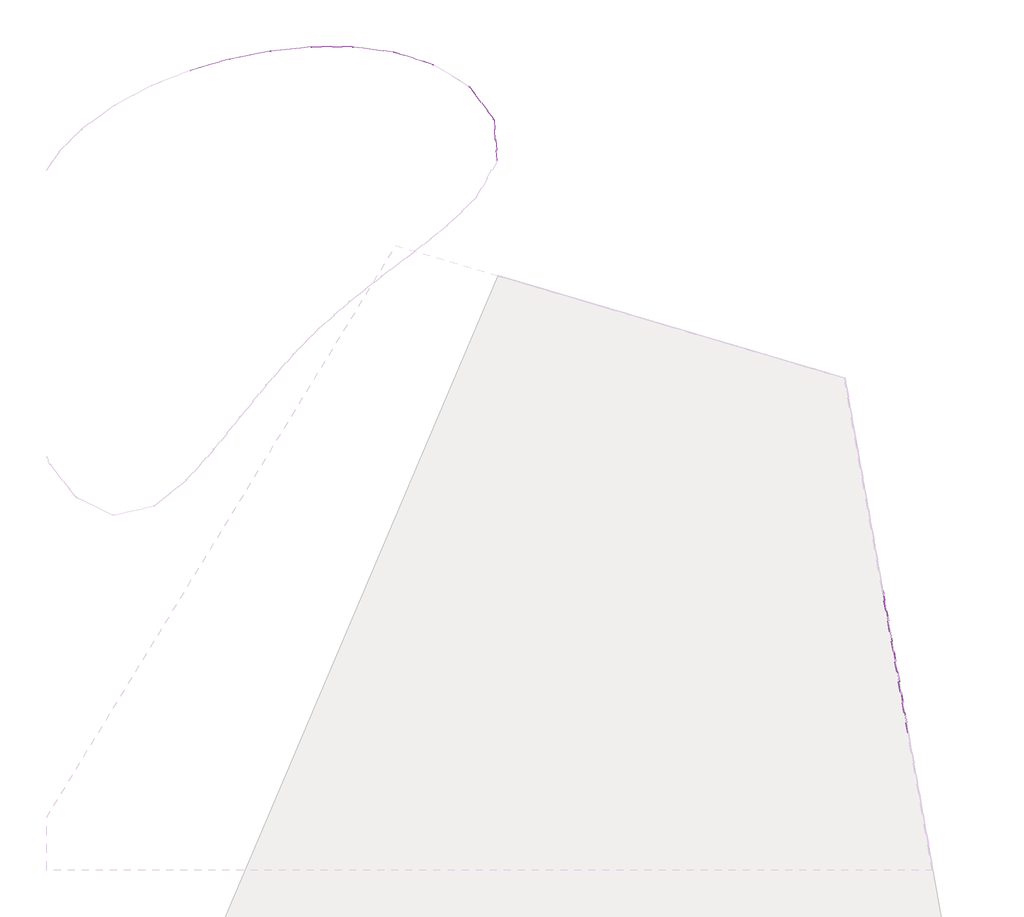
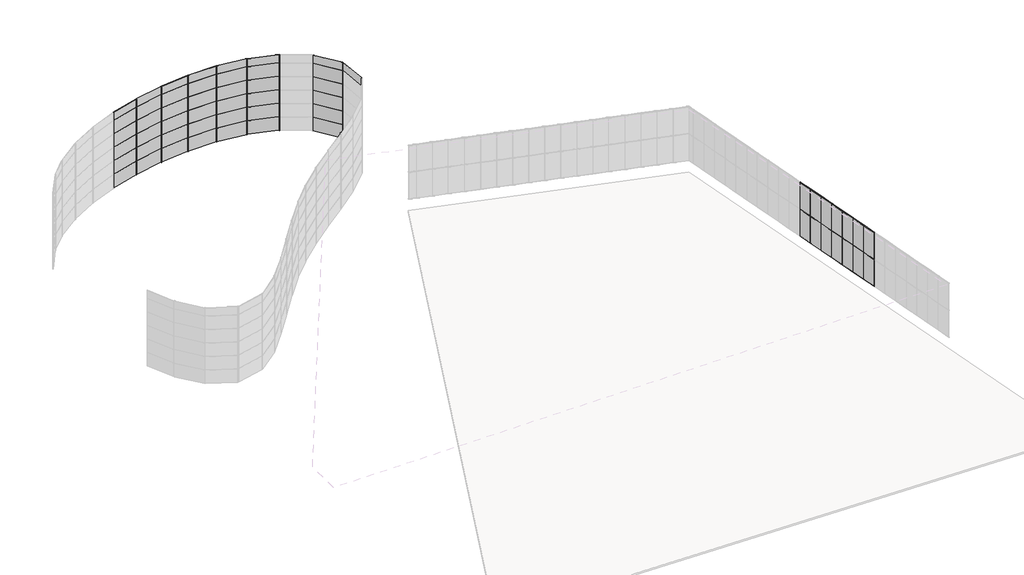
# One storey, part 7 of 8: 63 members, 57 plates.
"""IFC4 building model written with IfcOpenShell, lengths in millimetres."""

import ifcopenshell
import ifcopenshell.guid

model = None  # the IFC model being written
_history = None  # IfcOwnerHistory: only IFC2X3 demands one
_inside = {}  # id of a spatial element -> (the spatial element, [elements in it])
_under = {}  # id of a project, library or spatial element -> (it, [spatial elements below it])
_declared = {}  # id of a project -> (the project, [libraries it declares])
_typed = {}  # id of a type object -> (the type object, [elements of that type])
_made_of = {}  # id of a material, layer set ... -> (it, [elements and type objects made of it])


def new_model(schema):
    """Start an empty IFC model of exactly this schema.

    Asked for "IFC4X3", IfcOpenShell would pick the latest addendum, in which some entities
    have other attributes; the version numbers below select the first issue.
    IFC2X3 requires an IfcOwnerHistory on every rooted entity: one is made here for all.
    """
    global model, _history
    if schema == "IFC4X3":
        model = ifcopenshell.file(schema_version=(4, 3, 0, 0))
    else:
        model = ifcopenshell.file(schema=schema)
    _inside.clear()
    _under.clear()
    _declared.clear()
    _typed.clear()
    _made_of.clear()
    _history = None
    if model.schema == "IFC2X3":
        org = make("IfcOrganization", Name="unknown")
        user = make(
            "IfcPersonAndOrganization",
            ThePerson=make("IfcPerson", FamilyName="unknown"),
            TheOrganization=org,
        )
        app = make(
            "IfcApplication",
            ApplicationDeveloper=org,
            Version="unknown",
            ApplicationFullName="unknown",
            ApplicationIdentifier="unknown",
        )
        _history = make(
            "IfcOwnerHistory",
            OwningUser=user,
            OwningApplication=app,
            ChangeAction="ADDED",
            CreationDate=0,
        )
    return model


def make(cls, **values):
    """One entity of the class cls with the attributes given. An attribute that is None is left unset."""
    return model.create_entity(
        cls, **{name: value for name, value in values.items() if value is not None}
    )


def rooted(cls, **values):
    """An entity with a GlobalId (a new one), such as an element, a storey or a relation."""
    return make(cls, GlobalId=ifcopenshell.guid.new(), OwnerHistory=_history, **values)


def si_unit(unit_type, name, prefix=None):
    """IfcSIUnit, for example si_unit("LENGTHUNIT", "METRE", prefix="MILLI")."""
    return make("IfcSIUnit", UnitType=unit_type, Prefix=prefix, Name=name)


def assignment(units):
    """IfcUnitAssignment: the units of a project."""
    return None if units is None else make("IfcUnitAssignment", Units=units)


def point(xyz):
    """IfcCartesianPoint."""
    return None if xyz is None else make("IfcCartesianPoint", Coordinates=xyz)


def direction(xyz):
    """IfcDirection."""
    return None if xyz is None else make("IfcDirection", DirectionRatios=xyz)


def frame(location, z_axis=None, x_axis=None):
    """IfcAxis2Placement3D, a coordinate frame: its origin and axes. An axis left out is left unset."""
    return make(
        "IfcAxis2Placement3D",
        Location=point(location),
        Axis=direction(z_axis),
        RefDirection=direction(x_axis),
    )


def frame_2d(location, x_axis=None):
    """IfcAxis2Placement2D, a coordinate frame in the plane: its origin and x axis."""
    return make(
        "IfcAxis2Placement2D", Location=point(location), RefDirection=direction(x_axis)
    )


def origin():
    """The frame at (0, 0, 0) with its axes left unset."""
    return frame((0.0, 0.0, 0.0))


def origin_with_axes():
    """The frame at (0, 0, 0) with the z axis (0, 0, 1) and the x axis (1, 0, 0) written out."""
    return frame((0.0, 0.0, 0.0), z_axis=(0.0, 0.0, 1.0), x_axis=(1.0, 0.0, 0.0))


def origin_2d():
    """The frame at (0, 0) in the plane with its x axis left unset."""
    return frame_2d((0.0, 0.0))


def place(relative_to, where):
    """IfcLocalPlacement: puts the frame where relative to a parent placement (None: the world)."""
    return make(
        "IfcLocalPlacement", PlacementRelTo=relative_to, RelativePlacement=where
    )


def context(
    kind, dimensions, precision=None, world=None, true_north=None, identifier=None
):
    """IfcGeometricRepresentationContext, for example the 3D "Model" context."""
    return make(
        "IfcGeometricRepresentationContext",
        ContextIdentifier=identifier,
        ContextType=kind,
        CoordinateSpaceDimension=dimensions,
        Precision=precision,
        WorldCoordinateSystem=world,
        TrueNorth=true_north,
    )


def project(units=None, contexts=None):
    """IfcProject with its units and contexts."""
    return rooted(
        "IfcProject",
        Name="project",
        RepresentationContexts=contexts,
        UnitsInContext=assignment(units),
    )


def spatial(cls, under=None, at=None, **own):
    """A site, building, storey or space (cls), placed at a placement, below another one or the project."""
    s = rooted(cls, ObjectPlacement=at, **own)
    if under is not None:
        _under.setdefault(under.id(), (under, []))[1].append(s)
    return s


def polyline(points):
    """IfcPolyline through the points."""
    return make("IfcPolyline", Points=[point(p) for p in points])


def circle_curve(where, radius):
    """IfcCircle in the frame where."""
    return make("IfcCircle", Position=where, Radius=radius)


def trimmed(basis, trim1, trim2, sense, master):
    """IfcTrimmedCurve: the piece of a basis curve between two trims."""
    return make(
        "IfcTrimmedCurve",
        BasisCurve=basis,
        Trim1=trim1,
        Trim2=trim2,
        SenseAgreement=sense,
        MasterRepresentation=master,
    )


def segment(curve, same_sense, transition):
    """IfcCompositeCurveSegment."""
    return make(
        "IfcCompositeCurveSegment",
        Transition=transition,
        SameSense=same_sense,
        ParentCurve=curve,
    )


def composite_curve(segments, self_intersect=None):
    """IfcCompositeCurve: segments joined end to end."""
    return make("IfcCompositeCurve", Segments=segments, SelfIntersect=self_intersect)


def outline(outer, holes=None, kind="AREA"):
    """IfcArbitraryClosedProfileDef: a profile drawn as a closed curve; with holes, ...WithVoids."""
    if holes is None:
        return make("IfcArbitraryClosedProfileDef", ProfileType=kind, OuterCurve=outer)
    return make(
        "IfcArbitraryProfileDefWithVoids",
        ProfileType=kind,
        OuterCurve=outer,
        InnerCurves=holes,
    )


def extrude(swept, where, along, depth):
    """IfcExtrudedAreaSolid: the profile swept, set in the frame where, extruded along a direction by depth."""
    return make(
        "IfcExtrudedAreaSolid",
        SweptArea=swept,
        Position=where,
        ExtrudedDirection=direction(along),
        Depth=depth,
    )


def shape(context_of_items, identifier, shape_type, items):
    """IfcShapeRepresentation: the items that make up one representation, for example the "Body"."""
    return make(
        "IfcShapeRepresentation",
        ContextOfItems=context_of_items,
        RepresentationIdentifier=identifier,
        RepresentationType=shape_type,
        Items=items,
    )


def source(mapping_origin, context_of_items, identifier, shape_type, items):
    """IfcRepresentationMap: a shape defined once, which mapped items show again and again."""
    return make(
        "IfcRepresentationMap",
        MappingOrigin=mapping_origin,
        MappedRepresentation=shape(context_of_items, identifier, shape_type, items),
    )


def transform(
    local_origin,
    x_axis=None,
    y_axis=None,
    z_axis=None,
    scale=None,
    scale2=None,
    scale3=None,
    uniform=True,
):
    """IfcCartesianTransformationOperator3D, or its non-uniform kind. x_axis, y_axis, z_axis: its Axis1, 2, 3."""
    if uniform:
        return make(
            "IfcCartesianTransformationOperator3D",
            Axis1=direction(x_axis),
            Axis2=direction(y_axis),
            LocalOrigin=point(local_origin),
            Scale=scale,
            Axis3=direction(z_axis),
        )
    return make(
        "IfcCartesianTransformationOperator3DnonUniform",
        Axis1=direction(x_axis),
        Axis2=direction(y_axis),
        LocalOrigin=point(local_origin),
        Scale=scale,
        Axis3=direction(z_axis),
        Scale2=scale2,
        Scale3=scale3,
    )


def mapped(mapping_source, mapping_target):
    """IfcMappedItem: shows the shape of a source again, moved by a transform."""
    return make(
        "IfcMappedItem", MappingSource=mapping_source, MappingTarget=mapping_target
    )


def made_of(thing, what):
    """Note that an element or type object is made of a material, layer set ...; save() writes the relation."""
    if what is not None:
        _made_of.setdefault(what.id(), (what, []))[1].append(thing)
    return thing


def element(
    cls,
    number,
    at=None,
    inside=None,
    cuts=None,
    type_object=None,
    material=None,
    context=None,
    identifier="Body",
    shape_type=None,
    held_by="IfcProductDefinitionShape",
    body=None,
    shapes=None,
    **own,
):
    """One element of the class cls, such as IfcWall. Its Tag is "e" and its number.

    at: its placement. inside: the storey or other place that contains it. cuts: it is an
    opening in that element (IfcRelVoidsElement). A single representation is given by context,
    identifier, shape_type and body (its items); several are given by shapes. held_by: the class
    of the entity that holds the representations. save() writes the other relations.
    """
    e = rooted(cls, Tag="e%d" % number, ObjectPlacement=at, **own)
    if body is not None:
        shapes = [shape(context, identifier, shape_type, body)]
    if shapes is not None:
        e.Representation = make(held_by, Representations=shapes)
    if inside is not None:
        _inside.setdefault(inside.id(), (inside, []))[1].append(e)
    if cuts is not None:
        rooted(
            "IfcRelVoidsElement", RelatingBuildingElement=cuts, RelatedOpeningElement=e
        )
    if type_object is not None:
        _typed.setdefault(type_object.id(), (type_object, []))[1].append(e)
    return made_of(e, material)


def aggregate(whole, parts):
    """IfcRelAggregates: a whole, such as a stair, and the parts it consists of."""
    return rooted("IfcRelAggregates", RelatingObject=whole, RelatedObjects=parts)


def save(model, path):
    """Write the relations noted so far, then the file.

    IfcRelAggregates (storeys below a building ...), IfcRelContainedInSpatialStructure (elements
    in a storey), IfcRelDefinesByType, IfcRelAssociatesMaterial and IfcRelDeclares: one each for
    every whole, place, type object, material and project.
    """
    for whole, parts in _under.values():
        aggregate(whole, parts)
    for where, things in _inside.values():
        rooted(
            "IfcRelContainedInSpatialStructure",
            RelatedElements=things,
            RelatingStructure=where,
        )
    for kind, things in _typed.values():
        rooted("IfcRelDefinesByType", RelatedObjects=things, RelatingType=kind)
    for what, things in _made_of.values():
        rooted("IfcRelAssociatesMaterial", RelatedObjects=things, RelatingMaterial=what)
    for by, libraries in _declared.values():
        rooted("IfcRelDeclares", RelatingContext=by, RelatedDefinitions=libraries)
    model.write(path)


def montante_circular_25_mm_raio_ce826986(model_context):
    return source(origin(), model_context, "Body", "SweptSolid", [
        extrude(outline(composite_curve([segment(trimmed(circle_curve(frame_2d((-25.0, 0.0)), 25.0), [point((0.0, 0.0))], [point((-50.0, 0.0))], False, "CARTESIAN"), True, "CONTINUOUS"), segment(trimmed(circle_curve(frame_2d((-25.0, 0.0)), 25.0), [point((-50.0, 0.0))], [point((0.0, 0.0))], False, "CARTESIAN"), True, "CONTINUOUS")], self_intersect=False)), frame((0.0, 0.0, -1500.0), z_axis=(0.0, 0.0, 1.0), x_axis=(1.0, 0.0, 0.0)), (0.0, 0.0, 1.0), 1500.0),
    ])


def montante_circular_25_mm_raio_36e581cf(model_context):
    return source(origin(), model_context, "Body", "SweptSolid", [
        extrude(outline(composite_curve([segment(trimmed(circle_curve(origin_2d(), 25.0), [point((25.0, 0.0))], [point((-25.0, 0.0))], False, "CARTESIAN"), True, "CONTINUOUS"), segment(trimmed(circle_curve(origin_2d(), 25.0), [point((-25.0, 0.0))], [point((25.0, 0.0))], False, "CARTESIAN"), True, "CONTINUOUS")], self_intersect=False)), frame((0.0, 0.0, -1500.0), z_axis=(0.0, 0.0, 1.0), x_axis=(1.0, 0.0, 0.0)), (0.0, 0.0, 1.0), 1500.0),
    ])


def montante_circular_25_mm_raio_8ba79aec(model_context):
    return source(origin(), model_context, "Body", "SweptSolid", [
        extrude(outline(composite_curve([segment(trimmed(circle_curve(origin_2d(), 25.0), [point((25.0, 0.0))], [point((-25.0, 0.0))], False, "CARTESIAN"), True, "CONTINUOUS"), segment(trimmed(circle_curve(origin_2d(), 25.0), [point((-25.0, 0.0))], [point((25.0, 0.0))], False, "CARTESIAN"), True, "CONTINUOUS")], self_intersect=False)), frame((0.0, 0.0, -900.0), z_axis=(0.0, 0.0, 1.0), x_axis=(1.0, 0.0, 0.0)), (0.0, 0.0, 1.0), 900.0),
    ])


def painel_do_sistema_5ef9eced(model_context):
    return source(origin(), model_context, "Body", "SweptSolid", [
        extrude(outline(polyline([(1475.0, 24.5), (-1475.0, 24.5), (-1475.0, 49.5), (1475.0, 49.5), (1475.0, 24.5)])), origin_with_axes(), (0.0, 0.0, 1.0), 1500.0),
    ])


def painel_do_sistema_85ccde5d(model_context):
    return source(origin(), model_context, "Body", "SweptSolid", [
        extrude(outline(polyline([(1475.0, -49.5), (-1475.0, -49.5), (-1475.0, -24.5), (1475.0, -24.5), (1475.0, -49.5)])), origin_with_axes(), (0.0, 0.0, 1.0), 1500.0),
    ])


def painel_do_sistema_d8fd150b(model_context):
    return source(origin(), model_context, "Body", "SweptSolid", [
        extrude(outline(polyline([(1475.0, -49.5), (-1475.0, -49.5), (-1475.0, -24.5), (1475.0, -24.5), (1475.0, -49.5)])), origin_with_axes(), (0.0, 0.0, 1.0), 900.0),
    ])


def painel_do_sistema_af596b93(model_context):
    return source(origin(), model_context, "Body", "SweptSolid", [
        extrude(outline(polyline([(1462.4999925, 24.5), (-1462.4999925, 24.5), (-1462.4999925, 49.5), (1462.4999925, 49.5), (1462.4999925, 24.5)])), origin_with_axes(), (0.0, 0.0, 1.0), 1500.0),
    ])


model = new_model("IFC4")

# Units and contexts
model_context = context("Model", 3, world=origin())
ifc_project = project(units=[si_unit("LENGTHUNIT", "METRE", prefix="MILLI")], contexts=[model_context])

# Site, building, storey
site = spatial("IfcSite", under=ifc_project)
building = spatial("IfcBuilding", under=site)
storey = spatial("IfcBuildingStorey", under=building, Name="Nível 3", Elevation=7695.2)

# Members
placement = place(None, origin())
montante_circular_25_mm_raio_shape = montante_circular_25_mm_raio_ce826986(model_context)
element("IfcMember", 1, ObjectType="Montante circular : 25 mm Raio", at=placement, inside=storey, context=model_context, shape_type="MappedRepresentation", body=[
    mapped(montante_circular_25_mm_raio_shape, transform((22977.759166, 1270.3057737, 15000.0), x_axis=(0.0, 0.0, 1.0), y_axis=(0.9843520034862604, 0.17621331740985194, 0.0), z_axis=(-0.17621331740985194, 0.9843520034862604, 0.0))),
])
element("IfcMember", 2, ObjectType="Montante circular : 25 mm Raio", at=placement, inside=storey, context=model_context, shape_type="MappedRepresentation", body=[
    mapped(montante_circular_25_mm_raio_shape, transform((22713.4391899, 2746.833779, 15000.0), x_axis=(0.0, 0.0, 1.0), y_axis=(0.9843520034862615, 0.17621331740984614, 0.0), z_axis=(-0.1762133174098461, 0.9843520034862614, 0.0))),
])
element("IfcMember", 3, ObjectType="Montante circular : 25 mm Raio", at=placement, inside=storey, context=model_context, shape_type="MappedRepresentation", body=[
    mapped(montante_circular_25_mm_raio_shape, transform((22449.1192138, 4223.3617842, 15000.0), x_axis=(0.0, 0.0, 1.0), y_axis=(0.9843520034862611, 0.17621331740984805, 0.0), z_axis=(-0.17621331740984805, 0.9843520034862611, 0.0))),
])
element("IfcMember", 4, ObjectType="Montante circular : 25 mm Raio", at=placement, inside=storey, context=model_context, shape_type="MappedRepresentation", body=[
    mapped(montante_circular_25_mm_raio_shape, transform((22184.7992376, 5699.8897894, 15000.0), x_axis=(0.0, 0.0, 1.0), y_axis=(0.9843520034862614, 0.17621331740984636, 0.0), z_axis=(-0.17621331740984636, 0.9843520034862614, 0.0))),
])
element("IfcMember", 5, ObjectType="Montante circular : 25 mm Raio", at=placement, inside=storey, context=model_context, shape_type="MappedRepresentation", body=[
    mapped(montante_circular_25_mm_raio_shape, transform((21920.4792615, 7176.4177946, 15000.0), x_axis=(0.0, 0.0, 1.0), y_axis=(0.9843520034862608, 0.17621331740984977, 0.0), z_axis=(-0.17621331740984977, 0.9843520034862608, 0.0))),
])
element("IfcMember", 6, ObjectType="Montante circular : 25 mm Raio", at=placement, inside=storey, context=model_context, shape_type="MappedRepresentation", body=[
    mapped(montante_circular_25_mm_raio_shape, transform((21656.1592854, 8652.9457999, 15000.0), x_axis=(0.0, 0.0, 1.0), y_axis=(0.9843520034862612, 0.17621331740984747, 0.0), z_axis=(-0.17621331740984747, 0.9843520034862612, 0.0))),
])
element("IfcMember", 7, ObjectType="Montante circular : 25 mm Raio", at=placement, inside=storey, context=model_context, shape_type="MappedRepresentation", body=[
    mapped(montante_circular_25_mm_raio_shape, transform((21391.8393093, 10129.4738051, 15000.0), x_axis=(0.0, 0.0, 1.0), y_axis=(0.9843520034862608, 0.17621331740984966, 0.0), z_axis=(-0.17621331740984966, 0.9843520034862608, 0.0))),
])
montante_circular_25_mm_raio_2_shape = montante_circular_25_mm_raio_36e581cf(model_context)
element("IfcMember", 8, ObjectType="Montante circular : 25 mm Raio", at=placement, inside=storey, context=model_context, shape_type="MappedRepresentation", body=[
    mapped(montante_circular_25_mm_raio_2_shape, transform((22977.759166, 1270.3057737, 9000.000015), x_axis=(0.0, 0.0, 1.0), y_axis=(0.9843520034862604, 0.17621331740985194, 0.0), z_axis=(-0.17621331740985194, 0.9843520034862604, 0.0))),
])
element("IfcMember", 9, ObjectType="Montante circular : 25 mm Raio", at=placement, inside=storey, context=model_context, shape_type="MappedRepresentation", body=[
    mapped(montante_circular_25_mm_raio_2_shape, transform((22713.4391899, 2746.833779, 9000.000015), x_axis=(0.0, 0.0, 1.0), y_axis=(0.9843520034862615, 0.17621331740984614, 0.0), z_axis=(-0.1762133174098461, 0.9843520034862614, 0.0))),
])
element("IfcMember", 10, ObjectType="Montante circular : 25 mm Raio", at=placement, inside=storey, context=model_context, shape_type="MappedRepresentation", body=[
    mapped(montante_circular_25_mm_raio_2_shape, transform((22449.1192138, 4223.3617842, 9000.000015), x_axis=(0.0, 0.0, 1.0), y_axis=(0.9843520034862611, 0.17621331740984805, 0.0), z_axis=(-0.17621331740984805, 0.9843520034862611, 0.0))),
])
element("IfcMember", 11, ObjectType="Montante circular : 25 mm Raio", at=placement, inside=storey, context=model_context, shape_type="MappedRepresentation", body=[
    mapped(montante_circular_25_mm_raio_2_shape, transform((22184.7992376, 5699.8897894, 9000.000015), x_axis=(0.0, 0.0, 1.0), y_axis=(0.9843520034862614, 0.17621331740984636, 0.0), z_axis=(-0.17621331740984636, 0.9843520034862614, 0.0))),
])
element("IfcMember", 12, ObjectType="Montante circular : 25 mm Raio", at=placement, inside=storey, context=model_context, shape_type="MappedRepresentation", body=[
    mapped(montante_circular_25_mm_raio_2_shape, transform((21920.4792615, 7176.4177946, 9000.000015), x_axis=(0.0, 0.0, 1.0), y_axis=(0.9843520034862608, 0.17621331740984977, 0.0), z_axis=(-0.17621331740984977, 0.9843520034862608, 0.0))),
])
element("IfcMember", 13, ObjectType="Montante circular : 25 mm Raio", at=placement, inside=storey, context=model_context, shape_type="MappedRepresentation", body=[
    mapped(montante_circular_25_mm_raio_2_shape, transform((21656.1592854, 8652.9457999, 9000.000015), x_axis=(0.0, 0.0, 1.0), y_axis=(0.9843520034862612, 0.17621331740984775, 0.0), z_axis=(-0.17621331740984772, 0.9843520034862611, 0.0))),
])
element("IfcMember", 14, ObjectType="Montante circular : 25 mm Raio", at=placement, inside=storey, context=model_context, shape_type="MappedRepresentation", body=[
    mapped(montante_circular_25_mm_raio_2_shape, transform((21391.8393093, 10129.4738051, 9000.000015), x_axis=(0.0, 0.0, 1.0), y_axis=(0.9843520034862608, 0.17621331740984966, 0.0), z_axis=(-0.17621331740984966, 0.9843520034862608, 0.0))),
])
element("IfcMember", 15, ObjectType="Montante circular : 25 mm Raio", at=placement, inside=storey, context=model_context, shape_type="MappedRepresentation", body=[
    mapped(montante_circular_25_mm_raio_2_shape, transform((22977.759166, 1270.3057737, 12000.000015), x_axis=(0.0, 0.0, 1.0), y_axis=(0.9843520034862604, 0.17621331740985194, 0.0), z_axis=(-0.17621331740985194, 0.9843520034862604, 0.0))),
])
element("IfcMember", 16, ObjectType="Montante circular : 25 mm Raio", at=placement, inside=storey, context=model_context, shape_type="MappedRepresentation", body=[
    mapped(montante_circular_25_mm_raio_2_shape, transform((22713.4391899, 2746.833779, 12000.000015), x_axis=(0.0, 0.0, 1.0), y_axis=(0.9843520034862615, 0.17621331740984614, 0.0), z_axis=(-0.1762133174098461, 0.9843520034862614, 0.0))),
])
element("IfcMember", 17, ObjectType="Montante circular : 25 mm Raio", at=placement, inside=storey, context=model_context, shape_type="MappedRepresentation", body=[
    mapped(montante_circular_25_mm_raio_2_shape, transform((22449.1192138, 4223.3617842, 12000.000015), x_axis=(0.0, 0.0, 1.0), y_axis=(0.9843520034862611, 0.1762133174098481, 0.0), z_axis=(-0.1762133174098481, 0.9843520034862611, 0.0))),
])
element("IfcMember", 18, ObjectType="Montante circular : 25 mm Raio", at=placement, inside=storey, context=model_context, shape_type="MappedRepresentation", body=[
    mapped(montante_circular_25_mm_raio_2_shape, transform((22184.7992376, 5699.8897894, 12000.000015), x_axis=(0.0, 0.0, 1.0), y_axis=(0.9843520034862614, 0.17621331740984636, 0.0), z_axis=(-0.17621331740984636, 0.9843520034862614, 0.0))),
])
element("IfcMember", 19, ObjectType="Montante circular : 25 mm Raio", at=placement, inside=storey, context=model_context, shape_type="MappedRepresentation", body=[
    mapped(montante_circular_25_mm_raio_2_shape, transform((21920.4792615, 7176.4177946, 12000.000015), x_axis=(0.0, 0.0, 1.0), y_axis=(0.9843520034862608, 0.17621331740984977, 0.0), z_axis=(-0.17621331740984977, 0.9843520034862608, 0.0))),
])
element("IfcMember", 20, ObjectType="Montante circular : 25 mm Raio", at=placement, inside=storey, context=model_context, shape_type="MappedRepresentation", body=[
    mapped(montante_circular_25_mm_raio_2_shape, transform((21656.1592854, 8652.9457999, 12000.000015), x_axis=(0.0, 0.0, 1.0), y_axis=(0.9843520034862612, 0.17621331740984775, 0.0), z_axis=(-0.17621331740984772, 0.9843520034862611, 0.0))),
])
element("IfcMember", 21, ObjectType="Montante circular : 25 mm Raio", at=placement, inside=storey, context=model_context, shape_type="MappedRepresentation", body=[
    mapped(montante_circular_25_mm_raio_2_shape, transform((21391.8393093, 10129.4738051, 12000.000015), x_axis=(0.0, 0.0, 1.0), y_axis=(0.9843520034862608, 0.17621331740984966, 0.0), z_axis=(-0.17621331740984966, 0.9843520034862608, 0.0))),
])
element("IfcMember", 22, ObjectType="Montante circular : 25 mm Raio", at=placement, inside=storey, context=model_context, shape_type="MappedRepresentation", body=[
    mapped(montante_circular_25_mm_raio_2_shape, transform((-6868.5829053, 44343.271676, 9000.0), x_axis=(-0.3894872634933398, 0.9210318515537178, 0.0), y_axis=(0.9210318515537178, 0.3894872634933398, 0.0), z_axis=(0.0, 0.0, -1.0))),
])
element("IfcMember", 23, ObjectType="Montante circular : 25 mm Raio", at=placement, inside=storey, context=model_context, shape_type="MappedRepresentation", body=[
    mapped(montante_circular_25_mm_raio_2_shape, transform((-11244.034472, 48297.0103794, 9000.0), x_axis=(-0.9160451113541028, 0.40107524725947563, 0.0), y_axis=(0.40107524725947563, 0.9160451113541028, 0.0), z_axis=(0.0, 0.0, -1.0))),
])
element("IfcMember", 24, ObjectType="Montante circular : 25 mm Raio", at=placement, inside=storey, context=model_context, shape_type="MappedRepresentation", body=[
    mapped(montante_circular_25_mm_raio_2_shape, transform((-14105.1754803, 49199.1589981, 9000.0), x_axis=(-0.9782677823869713, 0.20734547485700608, 0.0), y_axis=(0.20734547485700608, 0.9782677823869713, 0.0), z_axis=(0.0, 0.0, -1.0))),
])
element("IfcMember", 25, ObjectType="Montante circular : 25 mm Raio", at=placement, inside=storey, context=model_context, shape_type="MappedRepresentation", body=[
    mapped(montante_circular_25_mm_raio_2_shape, transform((-17080.2416106, 49585.140242, 9000.0), x_axis=(-0.998380379517221, 0.0568912804834772, 0.0), y_axis=(0.0568912804834772, 0.998380379517221, 0.0), z_axis=(0.0, 0.0, -1.0))),
])
element("IfcMember", 26, ObjectType="Montante circular : 25 mm Raio", at=placement, inside=storey, context=model_context, shape_type="MappedRepresentation", body=[
    mapped(montante_circular_25_mm_raio_2_shape, transform((-20080.239517, 49581.5960042, 9000.0), x_axis=(-0.9985092878419478, -0.05458206750725284, 0.0), y_axis=(-0.05458206750725284, 0.9985092878419478, 0.0), z_axis=(0.0, 0.0, -1.0))),
])
element("IfcMember", 27, ObjectType="Montante circular : 25 mm Raio", at=placement, inside=storey, context=model_context, shape_type="MappedRepresentation", body=[
    mapped(montante_circular_25_mm_raio_2_shape, transform((-23064.637889, 49276.0369149, 9000.0), x_axis=(-0.9891120775870231, -0.14716418712269272, 0.0), y_axis=(-0.14716418712269272, 0.9891120775870231, 0.0), z_axis=(0.0, 0.0, -1.0))),
])
element("IfcMember", 28, ObjectType="Montante circular : 25 mm Raio", at=placement, inside=storey, context=model_context, shape_type="MappedRepresentation", body=[
    mapped(montante_circular_25_mm_raio_2_shape, transform((-26009.7169515, 48704.6269783, 9000.0), x_axis=(-0.9724041864044524, -0.23330258949076224, 0.0), y_axis=(-0.23330258949076224, 0.9724041864044524, 0.0), z_axis=(0.0, 0.0, -1.0))),
])
element("IfcMember", 29, ObjectType="Montante circular : 25 mm Raio", at=placement, inside=storey, context=model_context, shape_type="MappedRepresentation", body=[
    mapped(montante_circular_25_mm_raio_2_shape, transform((-6868.5829053, 44343.271676, 10500.0), x_axis=(-0.38948726349333973, 0.9210318515537178, 0.0), y_axis=(0.9210318515537178, 0.38948726349333973, 0.0), z_axis=(0.0, 0.0, -1.0))),
])
element("IfcMember", 30, ObjectType="Montante circular : 25 mm Raio", at=placement, inside=storey, context=model_context, shape_type="MappedRepresentation", body=[
    mapped(montante_circular_25_mm_raio_2_shape, transform((-11244.034472, 48297.0103794, 10500.0), x_axis=(-0.9160451113541028, 0.40107524725947563, 0.0), y_axis=(0.40107524725947563, 0.9160451113541028, 0.0), z_axis=(0.0, 0.0, -1.0))),
])
element("IfcMember", 31, ObjectType="Montante circular : 25 mm Raio", at=placement, inside=storey, context=model_context, shape_type="MappedRepresentation", body=[
    mapped(montante_circular_25_mm_raio_2_shape, transform((-14105.1754803, 49199.1589981, 10500.0), x_axis=(-0.9782677823869713, 0.20734547485700608, 0.0), y_axis=(0.20734547485700608, 0.9782677823869713, 0.0), z_axis=(0.0, 0.0, -1.0))),
])
element("IfcMember", 32, ObjectType="Montante circular : 25 mm Raio", at=placement, inside=storey, context=model_context, shape_type="MappedRepresentation", body=[
    mapped(montante_circular_25_mm_raio_2_shape, transform((-17080.2416106, 49585.140242, 10500.0), x_axis=(-0.998380379517221, 0.05689128048347741, 0.0), y_axis=(0.05689128048347741, 0.998380379517221, 0.0), z_axis=(0.0, 0.0, -1.0))),
])
element("IfcMember", 33, ObjectType="Montante circular : 25 mm Raio", at=placement, inside=storey, context=model_context, shape_type="MappedRepresentation", body=[
    mapped(montante_circular_25_mm_raio_2_shape, transform((-20080.239517, 49581.5960042, 10500.0), x_axis=(-0.9985092878419478, -0.05458206750725284, 0.0), y_axis=(-0.05458206750725284, 0.9985092878419478, 0.0), z_axis=(0.0, 0.0, -1.0))),
])
element("IfcMember", 34, ObjectType="Montante circular : 25 mm Raio", at=placement, inside=storey, context=model_context, shape_type="MappedRepresentation", body=[
    mapped(montante_circular_25_mm_raio_2_shape, transform((-23064.637889, 49276.0369149, 10500.0), x_axis=(-0.989112077587023, -0.14716418712269302, 0.0), y_axis=(-0.14716418712269302, 0.989112077587023, 0.0), z_axis=(0.0, 0.0, -1.0))),
])
element("IfcMember", 35, ObjectType="Montante circular : 25 mm Raio", at=placement, inside=storey, context=model_context, shape_type="MappedRepresentation", body=[
    mapped(montante_circular_25_mm_raio_2_shape, transform((-26009.7169515, 48704.6269783, 10500.0), x_axis=(-0.9724041864044524, -0.23330258949076224, 0.0), y_axis=(-0.23330258949076224, 0.9724041864044524, 0.0), z_axis=(0.0, 0.0, -1.0))),
])
element("IfcMember", 36, ObjectType="Montante circular : 25 mm Raio", at=placement, inside=storey, context=model_context, shape_type="MappedRepresentation", body=[
    mapped(montante_circular_25_mm_raio_2_shape, transform((-6868.5829053, 44343.271676, 12000.0), x_axis=(-0.38948726349333973, 0.9210318515537178, 0.0), y_axis=(0.9210318515537178, 0.38948726349333973, 0.0), z_axis=(0.0, 0.0, -1.0))),
])
element("IfcMember", 37, ObjectType="Montante circular : 25 mm Raio", at=placement, inside=storey, context=model_context, shape_type="MappedRepresentation", body=[
    mapped(montante_circular_25_mm_raio_2_shape, transform((-11244.034472, 48297.0103794, 12000.0), x_axis=(-0.9160451113541028, 0.40107524725947563, 0.0), y_axis=(0.40107524725947563, 0.9160451113541028, 0.0), z_axis=(0.0, 0.0, -1.0))),
])
element("IfcMember", 38, ObjectType="Montante circular : 25 mm Raio", at=placement, inside=storey, context=model_context, shape_type="MappedRepresentation", body=[
    mapped(montante_circular_25_mm_raio_2_shape, transform((-14105.1754803, 49199.1589981, 12000.0), x_axis=(-0.9782677823869713, 0.20734547485700608, 0.0), y_axis=(0.20734547485700608, 0.9782677823869713, 0.0), z_axis=(0.0, 0.0, -1.0))),
])
element("IfcMember", 39, ObjectType="Montante circular : 25 mm Raio", at=placement, inside=storey, context=model_context, shape_type="MappedRepresentation", body=[
    mapped(montante_circular_25_mm_raio_2_shape, transform((-17080.2416106, 49585.140242, 12000.0), x_axis=(-0.998380379517221, 0.0568912804834772, 0.0), y_axis=(0.0568912804834772, 0.998380379517221, 0.0), z_axis=(0.0, 0.0, -1.0))),
])
element("IfcMember", 40, ObjectType="Montante circular : 25 mm Raio", at=placement, inside=storey, context=model_context, shape_type="MappedRepresentation", body=[
    mapped(montante_circular_25_mm_raio_2_shape, transform((-20080.239517, 49581.5960042, 12000.0), x_axis=(-0.9985092878419478, -0.05458206750725285, 0.0), y_axis=(-0.05458206750725285, 0.9985092878419478, 0.0), z_axis=(0.0, 0.0, -1.0))),
])
element("IfcMember", 41, ObjectType="Montante circular : 25 mm Raio", at=placement, inside=storey, context=model_context, shape_type="MappedRepresentation", body=[
    mapped(montante_circular_25_mm_raio_2_shape, transform((-23064.637889, 49276.0369149, 12000.0), x_axis=(-0.989112077587023, -0.14716418712269305, 0.0), y_axis=(-0.14716418712269305, 0.989112077587023, 0.0), z_axis=(0.0, 0.0, -1.0))),
])
element("IfcMember", 42, ObjectType="Montante circular : 25 mm Raio", at=placement, inside=storey, context=model_context, shape_type="MappedRepresentation", body=[
    mapped(montante_circular_25_mm_raio_2_shape, transform((-26009.7169515, 48704.6269783, 12000.0), x_axis=(-0.9724041864044525, -0.23330258949076174, 0.0), y_axis=(-0.23330258949076174, 0.9724041864044525, 0.0), z_axis=(0.0, 0.0, -1.0))),
])
element("IfcMember", 43, ObjectType="Montante circular : 25 mm Raio", at=placement, inside=storey, context=model_context, shape_type="MappedRepresentation", body=[
    mapped(montante_circular_25_mm_raio_2_shape, transform((-6868.5829053, 44343.271676, 13500.0), x_axis=(-0.3894872634933398, 0.9210318515537178, 0.0), y_axis=(0.9210318515537178, 0.3894872634933398, 0.0), z_axis=(0.0, 0.0, -1.0))),
])
element("IfcMember", 44, ObjectType="Montante circular : 25 mm Raio", at=placement, inside=storey, context=model_context, shape_type="MappedRepresentation", body=[
    mapped(montante_circular_25_mm_raio_2_shape, transform((-11244.034472, 48297.0103794, 13500.0), x_axis=(-0.9160451113541028, 0.40107524725947563, 0.0), y_axis=(0.40107524725947563, 0.9160451113541028, 0.0), z_axis=(0.0, 0.0, -1.0))),
])
element("IfcMember", 45, ObjectType="Montante circular : 25 mm Raio", at=placement, inside=storey, context=model_context, shape_type="MappedRepresentation", body=[
    mapped(montante_circular_25_mm_raio_2_shape, transform((-14105.1754803, 49199.1589981, 13500.0), x_axis=(-0.9782677823869713, 0.20734547485700608, 0.0), y_axis=(0.20734547485700608, 0.9782677823869713, 0.0), z_axis=(0.0, 0.0, -1.0))),
])
element("IfcMember", 46, ObjectType="Montante circular : 25 mm Raio", at=placement, inside=storey, context=model_context, shape_type="MappedRepresentation", body=[
    mapped(montante_circular_25_mm_raio_2_shape, transform((-17080.2416106, 49585.140242, 13500.0), x_axis=(-0.998380379517221, 0.0568912804834772, 0.0), y_axis=(0.0568912804834772, 0.998380379517221, 0.0), z_axis=(0.0, 0.0, -1.0))),
])
element("IfcMember", 47, ObjectType="Montante circular : 25 mm Raio", at=placement, inside=storey, context=model_context, shape_type="MappedRepresentation", body=[
    mapped(montante_circular_25_mm_raio_2_shape, transform((-20080.239517, 49581.5960042, 13500.0), x_axis=(-0.9985092878419478, -0.054582067507252835, 0.0), y_axis=(-0.054582067507252835, 0.9985092878419478, 0.0), z_axis=(0.0, 0.0, -1.0))),
])
element("IfcMember", 48, ObjectType="Montante circular : 25 mm Raio", at=placement, inside=storey, context=model_context, shape_type="MappedRepresentation", body=[
    mapped(montante_circular_25_mm_raio_2_shape, transform((-23064.637889, 49276.0369149, 13500.0), x_axis=(-0.9891120775870231, -0.14716418712269272, 0.0), y_axis=(-0.14716418712269272, 0.9891120775870231, 0.0), z_axis=(0.0, 0.0, -1.0))),
])
element("IfcMember", 49, ObjectType="Montante circular : 25 mm Raio", at=placement, inside=storey, context=model_context, shape_type="MappedRepresentation", body=[
    mapped(montante_circular_25_mm_raio_2_shape, transform((-26009.7169515, 48704.6269783, 13500.0), x_axis=(-0.9724041864044524, -0.23330258949076224, 0.0), y_axis=(-0.23330258949076224, 0.9724041864044524, 0.0), z_axis=(0.0, 0.0, -1.0))),
])
element("IfcMember", 50, ObjectType="Montante circular : 25 mm Raio", at=placement, inside=storey, context=model_context, shape_type="MappedRepresentation", body=[
    mapped(montante_circular_25_mm_raio_2_shape, transform((-6868.5829053, 44343.271676, 15000.0), x_axis=(-0.3894872634933398, 0.9210318515537178, 0.0), y_axis=(0.9210318515537178, 0.3894872634933398, 0.0), z_axis=(0.0, 0.0, -1.0))),
])
element("IfcMember", 51, ObjectType="Montante circular : 25 mm Raio", at=placement, inside=storey, context=model_context, shape_type="MappedRepresentation", body=[
    mapped(montante_circular_25_mm_raio_2_shape, transform((-11244.034472, 48297.0103794, 15000.0), x_axis=(-0.9160451113541028, 0.4010752472594757, 0.0), y_axis=(0.4010752472594757, 0.9160451113541028, 0.0), z_axis=(0.0, 0.0, -1.0))),
])
element("IfcMember", 52, ObjectType="Montante circular : 25 mm Raio", at=placement, inside=storey, context=model_context, shape_type="MappedRepresentation", body=[
    mapped(montante_circular_25_mm_raio_2_shape, transform((-14105.1754803, 49199.1589981, 15000.0), x_axis=(-0.9782677823869713, 0.20734547485700608, 0.0), y_axis=(0.20734547485700608, 0.9782677823869713, 0.0), z_axis=(0.0, 0.0, -1.0))),
])
element("IfcMember", 53, ObjectType="Montante circular : 25 mm Raio", at=placement, inside=storey, context=model_context, shape_type="MappedRepresentation", body=[
    mapped(montante_circular_25_mm_raio_2_shape, transform((-17080.2416106, 49585.140242, 15000.0), x_axis=(-0.998380379517221, 0.0568912804834772, 0.0), y_axis=(0.0568912804834772, 0.998380379517221, 0.0), z_axis=(0.0, 0.0, -1.0))),
])
element("IfcMember", 54, ObjectType="Montante circular : 25 mm Raio", at=placement, inside=storey, context=model_context, shape_type="MappedRepresentation", body=[
    mapped(montante_circular_25_mm_raio_2_shape, transform((-20080.239517, 49581.5960042, 15000.0), x_axis=(-0.9985092878419478, -0.05458206750725284, 0.0), y_axis=(-0.05458206750725284, 0.9985092878419478, 0.0), z_axis=(0.0, 0.0, -1.0))),
])
element("IfcMember", 55, ObjectType="Montante circular : 25 mm Raio", at=placement, inside=storey, context=model_context, shape_type="MappedRepresentation", body=[
    mapped(montante_circular_25_mm_raio_2_shape, transform((-23064.637889, 49276.0369149, 15000.0), x_axis=(-0.9891120775870231, -0.14716418712269272, 0.0), y_axis=(-0.14716418712269272, 0.9891120775870231, 0.0), z_axis=(0.0, 0.0, -1.0))),
])
element("IfcMember", 56, ObjectType="Montante circular : 25 mm Raio", at=placement, inside=storey, context=model_context, shape_type="MappedRepresentation", body=[
    mapped(montante_circular_25_mm_raio_2_shape, transform((-26009.7169515, 48704.6269783, 15000.0), x_axis=(-0.9724041864044524, -0.23330258949076224, 0.0), y_axis=(-0.23330258949076224, 0.9724041864044524, 0.0), z_axis=(0.0, 0.0, -1.0))),
])
montante_circular_25_mm_raio_3_shape = montante_circular_25_mm_raio_8ba79aec(model_context)
element("IfcMember", 57, ObjectType="Montante circular : 25 mm Raio", at=placement, inside=storey, context=model_context, shape_type="MappedRepresentation", body=[
    mapped(montante_circular_25_mm_raio_3_shape, transform((-6868.5829053, 44343.271676, 16500.0), x_axis=(-0.3894872634933398, 0.9210318515537178, 0.0), y_axis=(0.9210318515537178, 0.3894872634933398, 0.0), z_axis=(0.0, 0.0, -1.0))),
])
element("IfcMember", 58, ObjectType="Montante circular : 25 mm Raio", at=placement, inside=storey, context=model_context, shape_type="MappedRepresentation", body=[
    mapped(montante_circular_25_mm_raio_3_shape, transform((-11244.034472, 48297.0103794, 16500.0), x_axis=(-0.9160451113541028, 0.40107524725947563, 0.0), y_axis=(0.40107524725947563, 0.9160451113541028, 0.0), z_axis=(0.0, 0.0, -1.0))),
])
element("IfcMember", 59, ObjectType="Montante circular : 25 mm Raio", at=placement, inside=storey, context=model_context, shape_type="MappedRepresentation", body=[
    mapped(montante_circular_25_mm_raio_3_shape, transform((-14105.1754803, 49199.1589981, 16500.0), x_axis=(-0.9782677823869713, 0.20734547485700608, 0.0), y_axis=(0.20734547485700608, 0.9782677823869713, 0.0), z_axis=(0.0, 0.0, -1.0))),
])
element("IfcMember", 60, ObjectType="Montante circular : 25 mm Raio", at=placement, inside=storey, context=model_context, shape_type="MappedRepresentation", body=[
    mapped(montante_circular_25_mm_raio_3_shape, transform((-17080.2416106, 49585.140242, 16500.0), x_axis=(-0.998380379517221, 0.0568912804834772, 0.0), y_axis=(0.0568912804834772, 0.998380379517221, 0.0), z_axis=(0.0, 0.0, -1.0))),
])
element("IfcMember", 61, ObjectType="Montante circular : 25 mm Raio", at=placement, inside=storey, context=model_context, shape_type="MappedRepresentation", body=[
    mapped(montante_circular_25_mm_raio_3_shape, transform((-20080.239517, 49581.5960042, 16500.0), x_axis=(-0.9985092878419478, -0.05458206750725284, 0.0), y_axis=(-0.05458206750725284, 0.9985092878419478, 0.0), z_axis=(0.0, 0.0, -1.0))),
])
element("IfcMember", 62, ObjectType="Montante circular : 25 mm Raio", at=placement, inside=storey, context=model_context, shape_type="MappedRepresentation", body=[
    mapped(montante_circular_25_mm_raio_3_shape, transform((-23064.637889, 49276.0369149, 16500.0), x_axis=(-0.9891120775870231, -0.14716418712269266, 0.0), y_axis=(-0.14716418712269266, 0.9891120775870231, 0.0), z_axis=(0.0, 0.0, -1.0))),
])
element("IfcMember", 63, ObjectType="Montante circular : 25 mm Raio", at=placement, inside=storey, context=model_context, shape_type="MappedRepresentation", body=[
    mapped(montante_circular_25_mm_raio_3_shape, transform((-26009.7169515, 48704.6269783, 16500.0), x_axis=(-0.9724041864044524, -0.23330258949076224, 0.0), y_axis=(-0.23330258949076224, 0.9724041864044524, 0.0), z_axis=(0.0, 0.0, -1.0))),
])

# Plates
painel_do_sistema_shape = painel_do_sistema_5ef9eced(model_context)
element("IfcPlate", 64, ObjectType="Painel do sistema : Envidraçado", at=placement, inside=storey, context=model_context, shape_type="MappedRepresentation", body=[
    mapped(painel_do_sistema_shape, transform((22977.759166, 1270.3057737, 10500.000015), x_axis=(0.0, 0.0, 1.0), y_axis=(-0.9843520034862604, -0.17621331740985194, 0.0), z_axis=(0.17621331740985194, -0.9843520034862604, 0.0))),
])
element("IfcPlate", 65, ObjectType="Painel do sistema : Envidraçado", at=placement, inside=storey, context=model_context, shape_type="MappedRepresentation", body=[
    mapped(painel_do_sistema_shape, transform((22713.4391899, 2746.833779, 10500.000015), x_axis=(0.0, 0.0, 1.0), y_axis=(-0.9843520034862615, -0.1762133174098461, 0.0), z_axis=(0.1762133174098461, -0.9843520034862615, 0.0))),
])
element("IfcPlate", 66, ObjectType="Painel do sistema : Envidraçado", at=placement, inside=storey, context=model_context, shape_type="MappedRepresentation", body=[
    mapped(painel_do_sistema_shape, transform((22449.1192138, 4223.3617842, 10500.000015), x_axis=(0.0, 0.0, 1.0), y_axis=(-0.9843520034862611, -0.17621331740984814, 0.0), z_axis=(0.17621331740984814, -0.9843520034862611, 0.0))),
])
element("IfcPlate", 67, ObjectType="Painel do sistema : Envidraçado", at=placement, inside=storey, context=model_context, shape_type="MappedRepresentation", body=[
    mapped(painel_do_sistema_shape, transform((22184.7992376, 5699.8897894, 10500.000015), x_axis=(0.0, 0.0, 1.0), y_axis=(-0.9843520034862614, -0.17621331740984636, 0.0), z_axis=(0.17621331740984636, -0.9843520034862614, 0.0))),
])
element("IfcPlate", 68, ObjectType="Painel do sistema : Envidraçado", at=placement, inside=storey, context=model_context, shape_type="MappedRepresentation", body=[
    mapped(painel_do_sistema_shape, transform((21920.4792615, 7176.4177946, 10500.000015), x_axis=(0.0, 0.0, 1.0), y_axis=(-0.9843520034862608, -0.17621331740984977, 0.0), z_axis=(0.17621331740984977, -0.9843520034862608, 0.0))),
])
element("IfcPlate", 69, ObjectType="Painel do sistema : Envidraçado", at=placement, inside=storey, context=model_context, shape_type="MappedRepresentation", body=[
    mapped(painel_do_sistema_shape, transform((21656.1592854, 8652.9457999, 10500.000015), x_axis=(0.0, 0.0, 1.0), y_axis=(-0.9843520034862612, -0.17621331740984775, 0.0), z_axis=(0.17621331740984775, -0.9843520034862612, 0.0))),
])
element("IfcPlate", 70, ObjectType="Painel do sistema : Envidraçado", at=placement, inside=storey, context=model_context, shape_type="MappedRepresentation", body=[
    mapped(painel_do_sistema_shape, transform((21391.8393093, 10129.4738051, 10500.000015), x_axis=(0.0, 0.0, 1.0), y_axis=(-0.9843520034862608, -0.17621331740984963, 0.0), z_axis=(0.17621331740984963, -0.9843520034862608, 0.0))),
])
painel_do_sistema_2_shape = painel_do_sistema_85ccde5d(model_context)
element("IfcPlate", 71, ObjectType="Painel do sistema : Envidraçado", at=placement, inside=storey, context=model_context, shape_type="MappedRepresentation", body=[
    mapped(painel_do_sistema_2_shape, transform((-7777.0568462, 45536.8692208, 9000.0), x_axis=(-0.605649293912105, 0.7957316964805214, 0.0), y_axis=(-0.7957316964805214, -0.605649293912105, 0.0), z_axis=(0.0, 0.0, 1.0))),
])
element("IfcPlate", 72, ObjectType="Painel do sistema : Envidraçado", at=placement, inside=storey, context=model_context, shape_type="MappedRepresentation", body=[
    mapped(painel_do_sistema_2_shape, transform((-12674.6049762, 48748.0846888, 9000.0), x_axis=(-0.9537136694548437, 0.3007162062393331, 0.0), y_axis=(-0.3007162062393331, -0.9537136694548437, 0.0), z_axis=(0.0, 0.0, 1.0))),
])
element("IfcPlate", 73, ObjectType="Painel do sistema : Envidraçado", at=placement, inside=storey, context=model_context, shape_type="MappedRepresentation", body=[
    mapped(painel_do_sistema_2_shape, transform((-15592.7085455, 49392.1496201, 9000.0), x_axis=(-0.9916887100842772, 0.12866041462463337, 0.0), y_axis=(-0.12866041462463337, -0.9916887100842772, 0.0), z_axis=(0.0, 0.0, 1.0))),
])
element("IfcPlate", 74, ObjectType="Painel do sistema : Envidraçado", at=placement, inside=storey, context=model_context, shape_type="MappedRepresentation", body=[
    mapped(painel_do_sistema_2_shape, transform((-18580.2405638, 49583.3681231, 9000.0), x_axis=(-0.9999993021318769, -0.0011814126118296353, 0.0), y_axis=(0.0011814126118296353, -0.9999993021318769, 0.0), z_axis=(0.0, 0.0, 1.0))),
])
element("IfcPlate", 75, ObjectType="Painel do sistema : Envidraçado", at=placement, inside=storey, context=model_context, shape_type="MappedRepresentation", body=[
    mapped(painel_do_sistema_2_shape, transform((-21572.438703, 49428.8164595, 9000.0), x_axis=(-0.9947994573422398, -0.10185302976144209, 0.0), y_axis=(0.10185302976144209, -0.9947994573422398, 0.0), z_axis=(0.0, 0.0, 1.0))),
])
element("IfcPlate", 76, ObjectType="Painel do sistema : Envidraçado", at=placement, inside=storey, context=model_context, shape_type="MappedRepresentation", body=[
    mapped(painel_do_sistema_2_shape, transform((-24537.1774203, 48990.3319466, 9000.0), x_axis=(-0.9816930208347299, -0.19046997885331593, 0.0), y_axis=(0.19046997885331593, -0.9816930208347299, 0.0), z_axis=(0.0, 0.0, 1.0))),
])
element("IfcPlate", 77, ObjectType="Painel do sistema : Envidraçado", at=placement, inside=storey, context=model_context, shape_type="MappedRepresentation", body=[
    mapped(painel_do_sistema_2_shape, transform((-27451.1290162, 48289.4989741, 9000.0), x_axis=(-0.9609413764383952, -0.27675200279073414, 0.0), y_axis=(0.27675200279073414, -0.9609413764383952, 0.0), z_axis=(0.0, 0.0, 1.0))),
])
element("IfcPlate", 78, ObjectType="Painel do sistema : Envidraçado", at=placement, inside=storey, context=model_context, shape_type="MappedRepresentation", body=[
    mapped(painel_do_sistema_2_shape, transform((-7777.0568462, 45536.8692208, 10500.0), x_axis=(-0.605649293912105, 0.7957316964805214, 0.0), y_axis=(-0.7957316964805214, -0.605649293912105, 0.0), z_axis=(0.0, 0.0, 1.0))),
])
element("IfcPlate", 79, ObjectType="Painel do sistema : Envidraçado", at=placement, inside=storey, context=model_context, shape_type="MappedRepresentation", body=[
    mapped(painel_do_sistema_2_shape, transform((-12674.6049762, 48748.0846888, 10500.0), x_axis=(-0.9537136694548437, 0.3007162062393331, 0.0), y_axis=(-0.3007162062393331, -0.9537136694548437, 0.0), z_axis=(0.0, 0.0, 1.0))),
])
element("IfcPlate", 80, ObjectType="Painel do sistema : Envidraçado", at=placement, inside=storey, context=model_context, shape_type="MappedRepresentation", body=[
    mapped(painel_do_sistema_2_shape, transform((-15592.7085455, 49392.1496201, 10500.0), x_axis=(-0.9916887100842772, 0.12866041462463337, 0.0), y_axis=(-0.12866041462463337, -0.9916887100842772, 0.0), z_axis=(0.0, 0.0, 1.0))),
])
element("IfcPlate", 81, ObjectType="Painel do sistema : Envidraçado", at=placement, inside=storey, context=model_context, shape_type="MappedRepresentation", body=[
    mapped(painel_do_sistema_2_shape, transform((-18580.2405638, 49583.3681231, 10500.0), x_axis=(-0.9999993021318769, -0.0011814126118296353, 0.0), y_axis=(0.0011814126118296353, -0.9999993021318769, 0.0), z_axis=(0.0, 0.0, 1.0))),
])
element("IfcPlate", 82, ObjectType="Painel do sistema : Envidraçado", at=placement, inside=storey, context=model_context, shape_type="MappedRepresentation", body=[
    mapped(painel_do_sistema_2_shape, transform((-21572.438703, 49428.8164595, 10500.0), x_axis=(-0.9947994573422398, -0.10185302976144207, 0.0), y_axis=(0.10185302976144207, -0.9947994573422398, 0.0), z_axis=(0.0, 0.0, 1.0))),
])
element("IfcPlate", 83, ObjectType="Painel do sistema : Envidraçado", at=placement, inside=storey, context=model_context, shape_type="MappedRepresentation", body=[
    mapped(painel_do_sistema_2_shape, transform((-24537.1774203, 48990.3319466, 10500.0), x_axis=(-0.9816930208347299, -0.1904699788533159, 0.0), y_axis=(0.1904699788533159, -0.9816930208347299, 0.0), z_axis=(0.0, 0.0, 1.0))),
])
element("IfcPlate", 84, ObjectType="Painel do sistema : Envidraçado", at=placement, inside=storey, context=model_context, shape_type="MappedRepresentation", body=[
    mapped(painel_do_sistema_2_shape, transform((-27451.1290162, 48289.4989741, 10500.0), x_axis=(-0.9609413764383952, -0.27675200279073414, 0.0), y_axis=(0.27675200279073414, -0.9609413764383952, 0.0), z_axis=(0.0, 0.0, 1.0))),
])
element("IfcPlate", 85, ObjectType="Painel do sistema : Envidraçado", at=placement, inside=storey, context=model_context, shape_type="MappedRepresentation", body=[
    mapped(painel_do_sistema_2_shape, transform((-7777.0568462, 45536.8692208, 12000.0), x_axis=(-0.605649293912105, 0.7957316964805214, 0.0), y_axis=(-0.7957316964805214, -0.605649293912105, 0.0), z_axis=(0.0, 0.0, 1.0))),
])
element("IfcPlate", 86, ObjectType="Painel do sistema : Envidraçado", at=placement, inside=storey, context=model_context, shape_type="MappedRepresentation", body=[
    mapped(painel_do_sistema_2_shape, transform((-12674.6049762, 48748.0846888, 12000.0), x_axis=(-0.9537136694548437, 0.3007162062393331, 0.0), y_axis=(-0.3007162062393331, -0.9537136694548437, 0.0), z_axis=(0.0, 0.0, 1.0))),
])
element("IfcPlate", 87, ObjectType="Painel do sistema : Envidraçado", at=placement, inside=storey, context=model_context, shape_type="MappedRepresentation", body=[
    mapped(painel_do_sistema_2_shape, transform((-15592.7085455, 49392.1496201, 12000.0), x_axis=(-0.9916887100842772, 0.12866041462463337, 0.0), y_axis=(-0.12866041462463337, -0.9916887100842772, 0.0), z_axis=(0.0, 0.0, 1.0))),
])
element("IfcPlate", 88, ObjectType="Painel do sistema : Envidraçado", at=placement, inside=storey, context=model_context, shape_type="MappedRepresentation", body=[
    mapped(painel_do_sistema_2_shape, transform((-18580.2405638, 49583.3681231, 12000.0), x_axis=(-0.9999993021318769, -0.0011814126118296353, 0.0), y_axis=(0.0011814126118296353, -0.9999993021318769, 0.0), z_axis=(0.0, 0.0, 1.0))),
])
element("IfcPlate", 89, ObjectType="Painel do sistema : Envidraçado", at=placement, inside=storey, context=model_context, shape_type="MappedRepresentation", body=[
    mapped(painel_do_sistema_2_shape, transform((-21572.438703, 49428.8164595, 12000.0), x_axis=(-0.9947994573422398, -0.10185302976144207, 0.0), y_axis=(0.10185302976144207, -0.9947994573422398, 0.0), z_axis=(0.0, 0.0, 1.0))),
])
element("IfcPlate", 90, ObjectType="Painel do sistema : Envidraçado", at=placement, inside=storey, context=model_context, shape_type="MappedRepresentation", body=[
    mapped(painel_do_sistema_2_shape, transform((-24537.1774203, 48990.3319466, 12000.0), x_axis=(-0.9816930208347299, -0.1904699788533159, 0.0), y_axis=(0.1904699788533159, -0.9816930208347299, 0.0), z_axis=(0.0, 0.0, 1.0))),
])
element("IfcPlate", 91, ObjectType="Painel do sistema : Envidraçado", at=placement, inside=storey, context=model_context, shape_type="MappedRepresentation", body=[
    mapped(painel_do_sistema_2_shape, transform((-27451.1290162, 48289.4989741, 12000.0), x_axis=(-0.9609413764383952, -0.27675200279073414, 0.0), y_axis=(0.27675200279073414, -0.9609413764383952, 0.0), z_axis=(0.0, 0.0, 1.0))),
])
element("IfcPlate", 92, ObjectType="Painel do sistema : Envidraçado", at=placement, inside=storey, context=model_context, shape_type="MappedRepresentation", body=[
    mapped(painel_do_sistema_2_shape, transform((-7777.0568462, 45536.8692208, 13500.0), x_axis=(-0.605649293912105, 0.7957316964805214, 0.0), y_axis=(-0.7957316964805214, -0.605649293912105, 0.0), z_axis=(0.0, 0.0, 1.0))),
])
element("IfcPlate", 93, ObjectType="Painel do sistema : Envidraçado", at=placement, inside=storey, context=model_context, shape_type="MappedRepresentation", body=[
    mapped(painel_do_sistema_2_shape, transform((-12674.6049762, 48748.0846888, 13500.0), x_axis=(-0.9537136694548437, 0.3007162062393331, 0.0), y_axis=(-0.3007162062393331, -0.9537136694548437, 0.0), z_axis=(0.0, 0.0, 1.0))),
])
element("IfcPlate", 94, ObjectType="Painel do sistema : Envidraçado", at=placement, inside=storey, context=model_context, shape_type="MappedRepresentation", body=[
    mapped(painel_do_sistema_2_shape, transform((-15592.7085455, 49392.1496201, 13500.0), x_axis=(-0.9916887100842772, 0.12866041462463337, 0.0), y_axis=(-0.12866041462463337, -0.9916887100842772, 0.0), z_axis=(0.0, 0.0, 1.0))),
])
element("IfcPlate", 95, ObjectType="Painel do sistema : Envidraçado", at=placement, inside=storey, context=model_context, shape_type="MappedRepresentation", body=[
    mapped(painel_do_sistema_2_shape, transform((-18580.2405638, 49583.3681231, 13500.0), x_axis=(-0.9999993021318769, -0.0011814126118296353, 0.0), y_axis=(0.0011814126118296353, -0.9999993021318769, 0.0), z_axis=(0.0, 0.0, 1.0))),
])
element("IfcPlate", 96, ObjectType="Painel do sistema : Envidraçado", at=placement, inside=storey, context=model_context, shape_type="MappedRepresentation", body=[
    mapped(painel_do_sistema_2_shape, transform((-21572.438703, 49428.8164595, 13500.0), x_axis=(-0.9947994573422398, -0.10185302976144207, 0.0), y_axis=(0.10185302976144207, -0.9947994573422398, 0.0), z_axis=(0.0, 0.0, 1.0))),
])
element("IfcPlate", 97, ObjectType="Painel do sistema : Envidraçado", at=placement, inside=storey, context=model_context, shape_type="MappedRepresentation", body=[
    mapped(painel_do_sistema_2_shape, transform((-24537.1774203, 48990.3319466, 13500.0), x_axis=(-0.9816930208347299, -0.1904699788533159, 0.0), y_axis=(0.1904699788533159, -0.9816930208347299, 0.0), z_axis=(0.0, 0.0, 1.0))),
])
element("IfcPlate", 98, ObjectType="Painel do sistema : Envidraçado", at=placement, inside=storey, context=model_context, shape_type="MappedRepresentation", body=[
    mapped(painel_do_sistema_2_shape, transform((-27451.1290162, 48289.4989741, 13500.0), x_axis=(-0.9609413764383952, -0.27675200279073414, 0.0), y_axis=(0.27675200279073414, -0.9609413764383952, 0.0), z_axis=(0.0, 0.0, 1.0))),
])
element("IfcPlate", 99, ObjectType="Painel do sistema : Envidraçado", at=placement, inside=storey, context=model_context, shape_type="MappedRepresentation", body=[
    mapped(painel_do_sistema_2_shape, transform((-7777.0568462, 45536.8692208, 15000.0), x_axis=(-0.605649293912105, 0.7957316964805214, 0.0), y_axis=(-0.7957316964805214, -0.605649293912105, 0.0), z_axis=(0.0, 0.0, 1.0))),
])
element("IfcPlate", 100, ObjectType="Painel do sistema : Envidraçado", at=placement, inside=storey, context=model_context, shape_type="MappedRepresentation", body=[
    mapped(painel_do_sistema_2_shape, transform((-12674.6049762, 48748.0846888, 15000.0), x_axis=(-0.9537136694548437, 0.3007162062393331, 0.0), y_axis=(-0.3007162062393331, -0.9537136694548437, 0.0), z_axis=(0.0, 0.0, 1.0))),
])
element("IfcPlate", 101, ObjectType="Painel do sistema : Envidraçado", at=placement, inside=storey, context=model_context, shape_type="MappedRepresentation", body=[
    mapped(painel_do_sistema_2_shape, transform((-15592.7085455, 49392.1496201, 15000.0), x_axis=(-0.9916887100842772, 0.12866041462463337, 0.0), y_axis=(-0.12866041462463337, -0.9916887100842772, 0.0), z_axis=(0.0, 0.0, 1.0))),
])
element("IfcPlate", 102, ObjectType="Painel do sistema : Envidraçado", at=placement, inside=storey, context=model_context, shape_type="MappedRepresentation", body=[
    mapped(painel_do_sistema_2_shape, transform((-18580.2405638, 49583.3681231, 15000.0), x_axis=(-0.9999993021318769, -0.0011814126118296353, 0.0), y_axis=(0.0011814126118296353, -0.9999993021318769, 0.0), z_axis=(0.0, 0.0, 1.0))),
])
element("IfcPlate", 103, ObjectType="Painel do sistema : Envidraçado", at=placement, inside=storey, context=model_context, shape_type="MappedRepresentation", body=[
    mapped(painel_do_sistema_2_shape, transform((-21572.438703, 49428.8164595, 15000.0), x_axis=(-0.9947994573422398, -0.10185302976144207, 0.0), y_axis=(0.10185302976144207, -0.9947994573422398, 0.0), z_axis=(0.0, 0.0, 1.0))),
])
element("IfcPlate", 104, ObjectType="Painel do sistema : Envidraçado", at=placement, inside=storey, context=model_context, shape_type="MappedRepresentation", body=[
    mapped(painel_do_sistema_2_shape, transform((-24537.1774203, 48990.3319466, 15000.0), x_axis=(-0.9816930208347299, -0.1904699788533159, 0.0), y_axis=(0.1904699788533159, -0.9816930208347299, 0.0), z_axis=(0.0, 0.0, 1.0))),
])
element("IfcPlate", 105, ObjectType="Painel do sistema : Envidraçado", at=placement, inside=storey, context=model_context, shape_type="MappedRepresentation", body=[
    mapped(painel_do_sistema_2_shape, transform((-27451.1290162, 48289.4989741, 15000.0), x_axis=(-0.9609413764383952, -0.27675200279073414, 0.0), y_axis=(0.27675200279073414, -0.9609413764383952, 0.0), z_axis=(0.0, 0.0, 1.0))),
])
painel_do_sistema_3_shape = painel_do_sistema_d8fd150b(model_context)
element("IfcPlate", 106, ObjectType="Painel do sistema : Envidraçado", at=placement, inside=storey, context=model_context, shape_type="MappedRepresentation", body=[
    mapped(painel_do_sistema_3_shape, transform((-6748.0851686, 42848.1194111, 16500.0), x_axis=(-0.08033182448940979, 0.9967681766460056, 0.0), y_axis=(-0.9967681766460056, -0.08033182448940979, 0.0), z_axis=(0.0, 0.0, 1.0))),
])
element("IfcPlate", 107, ObjectType="Painel do sistema : Envidraçado", at=placement, inside=storey, context=model_context, shape_type="MappedRepresentation", body=[
    mapped(painel_do_sistema_3_shape, transform((-7777.0568462, 45536.8692208, 16500.0), x_axis=(-0.605649293912105, 0.7957316964805214, 0.0), y_axis=(-0.7957316964805214, -0.605649293912105, 0.0), z_axis=(0.0, 0.0, 1.0))),
])
element("IfcPlate", 108, ObjectType="Painel do sistema : Envidraçado", at=placement, inside=storey, context=model_context, shape_type="MappedRepresentation", body=[
    mapped(painel_do_sistema_3_shape, transform((-12674.6049762, 48748.0846888, 16500.0), x_axis=(-0.9537136694548437, 0.3007162062393331, 0.0), y_axis=(-0.3007162062393331, -0.9537136694548437, 0.0), z_axis=(0.0, 0.0, 1.0))),
])
element("IfcPlate", 109, ObjectType="Painel do sistema : Envidraçado", at=placement, inside=storey, context=model_context, shape_type="MappedRepresentation", body=[
    mapped(painel_do_sistema_3_shape, transform((-15592.7085455, 49392.1496201, 16500.0), x_axis=(-0.9916887100842772, 0.12866041462463337, 0.0), y_axis=(-0.12866041462463337, -0.9916887100842772, 0.0), z_axis=(0.0, 0.0, 1.0))),
])
element("IfcPlate", 110, ObjectType="Painel do sistema : Envidraçado", at=placement, inside=storey, context=model_context, shape_type="MappedRepresentation", body=[
    mapped(painel_do_sistema_3_shape, transform((-18580.2405638, 49583.3681231, 16500.0), x_axis=(-0.9999993021318769, -0.0011814126118296353, 0.0), y_axis=(0.0011814126118296353, -0.9999993021318769, 0.0), z_axis=(0.0, 0.0, 1.0))),
])
element("IfcPlate", 111, ObjectType="Painel do sistema : Envidraçado", at=placement, inside=storey, context=model_context, shape_type="MappedRepresentation", body=[
    mapped(painel_do_sistema_3_shape, transform((-21572.438703, 49428.8164595, 16500.0), x_axis=(-0.9947994573422398, -0.10185302976144209, 0.0), y_axis=(0.10185302976144209, -0.9947994573422398, 0.0), z_axis=(0.0, 0.0, 1.0))),
])
element("IfcPlate", 112, ObjectType="Painel do sistema : Envidraçado", at=placement, inside=storey, context=model_context, shape_type="MappedRepresentation", body=[
    mapped(painel_do_sistema_3_shape, transform((-24537.1774203, 48990.3319466, 16500.0), x_axis=(-0.9816930208347299, -0.1904699788533159, 0.0), y_axis=(0.1904699788533159, -0.9816930208347299, 0.0), z_axis=(0.0, 0.0, 1.0))),
])
element("IfcPlate", 113, ObjectType="Painel do sistema : Envidraçado", at=placement, inside=storey, context=model_context, shape_type="MappedRepresentation", body=[
    mapped(painel_do_sistema_3_shape, transform((-27451.1290162, 48289.4989741, 16500.0), x_axis=(-0.9609413764383952, -0.27675200279073414, 0.0), y_axis=(0.27675200279073414, -0.9609413764383952, 0.0), z_axis=(0.0, 0.0, 1.0))),
])
painel_do_sistema_4_shape = painel_do_sistema_af596b93(model_context)
element("IfcPlate", 114, ObjectType="Painel do sistema : Envidraçado", at=placement, inside=storey, context=model_context, shape_type="MappedRepresentation", body=[
    mapped(painel_do_sistema_4_shape, transform((22977.759166, 1270.3057737, 13487.5000075), x_axis=(0.0, 0.0, 1.0), y_axis=(-0.9843520034862604, -0.17621331740985197, 0.0), z_axis=(0.17621331740985197, -0.9843520034862604, 0.0))),
])
element("IfcPlate", 115, ObjectType="Painel do sistema : Envidraçado", at=placement, inside=storey, context=model_context, shape_type="MappedRepresentation", body=[
    mapped(painel_do_sistema_4_shape, transform((22713.4391899, 2746.833779, 13487.5000075), x_axis=(0.0, 0.0, 1.0), y_axis=(-0.9843520034862615, -0.1762133174098461, 0.0), z_axis=(0.1762133174098461, -0.9843520034862615, 0.0))),
])
element("IfcPlate", 116, ObjectType="Painel do sistema : Envidraçado", at=placement, inside=storey, context=model_context, shape_type="MappedRepresentation", body=[
    mapped(painel_do_sistema_4_shape, transform((22449.1192138, 4223.3617842, 13487.5000075), x_axis=(0.0, 0.0, 1.0), y_axis=(-0.9843520034862612, -0.17621331740984814, 0.0), z_axis=(0.17621331740984814, -0.9843520034862612, 0.0))),
])
element("IfcPlate", 117, ObjectType="Painel do sistema : Envidraçado", at=placement, inside=storey, context=model_context, shape_type="MappedRepresentation", body=[
    mapped(painel_do_sistema_4_shape, transform((22184.7992376, 5699.8897894, 13487.5000075), x_axis=(0.0, 0.0, 1.0), y_axis=(-0.9843520034862614, -0.17621331740984636, 0.0), z_axis=(0.17621331740984636, -0.9843520034862614, 0.0))),
])
element("IfcPlate", 118, ObjectType="Painel do sistema : Envidraçado", at=placement, inside=storey, context=model_context, shape_type="MappedRepresentation", body=[
    mapped(painel_do_sistema_4_shape, transform((21920.4792615, 7176.4177946, 13487.5000075), x_axis=(0.0, 0.0, 1.0), y_axis=(-0.9843520034862608, -0.17621331740984983, 0.0), z_axis=(0.17621331740984983, -0.9843520034862608, 0.0))),
])
element("IfcPlate", 119, ObjectType="Painel do sistema : Envidraçado", at=placement, inside=storey, context=model_context, shape_type="MappedRepresentation", body=[
    mapped(painel_do_sistema_4_shape, transform((21656.1592854, 8652.9457999, 13487.5000075), x_axis=(0.0, 0.0, 1.0), y_axis=(-0.9843520034862613, -0.1762133174098475, 0.0), z_axis=(0.1762133174098475, -0.9843520034862613, 0.0))),
])
element("IfcPlate", 120, ObjectType="Painel do sistema : Envidraçado", at=placement, inside=storey, context=model_context, shape_type="MappedRepresentation", body=[
    mapped(painel_do_sistema_4_shape, transform((21391.8393093, 10129.4738051, 13487.5000075), x_axis=(0.0, 0.0, 1.0), y_axis=(-0.9843520034862608, -0.17621331740984966, 0.0), z_axis=(0.17621331740984966, -0.9843520034862608, 0.0))),
])

save(model, "model.ifc")
